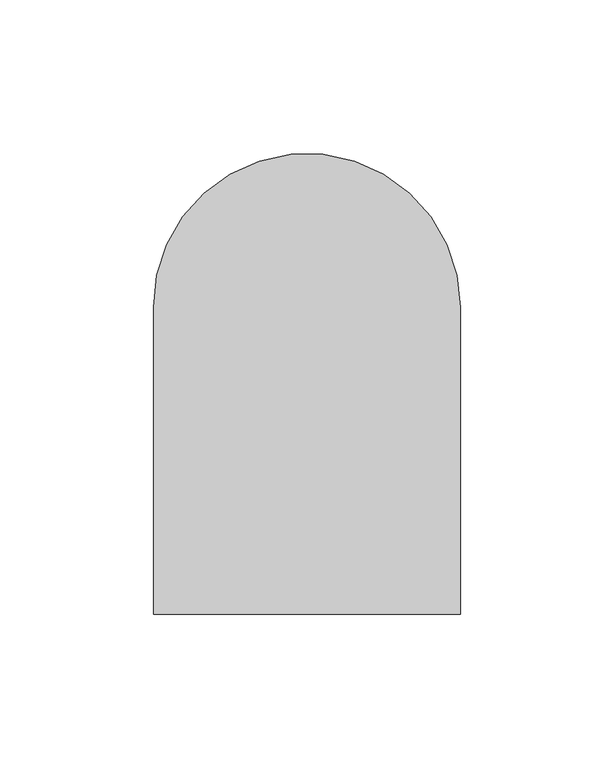
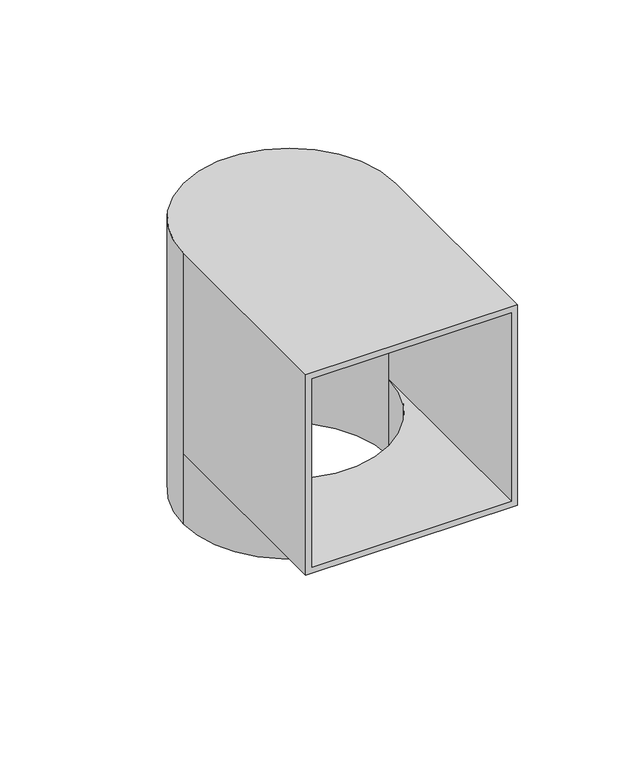
"""IFC4 building model written with IfcOpenShell, lengths in millimetres: proxy geometry, TN_Отвод угловой ТехноНИКОЛЬ : Отвод угловой, с квадратного сечения (100*100мм) в круглое (100мм)."""

import ifcopenshell
import ifcopenshell.guid

model = None  # the IFC model being written
_history = None  # IfcOwnerHistory: only IFC2X3 demands one
_inside = {}  # id of a spatial element -> (the spatial element, [elements in it])
_under = {}  # id of a project, library or spatial element -> (it, [spatial elements below it])
_declared = {}  # id of a project -> (the project, [libraries it declares])
_typed = {}  # id of a type object -> (the type object, [elements of that type])
_made_of = {}  # id of a material, layer set ... -> (it, [elements and type objects made of it])


def new_model(schema):
    """Start an empty IFC model of exactly this schema.

    Asked for "IFC4X3", IfcOpenShell would pick the latest addendum, in which some entities
    have other attributes; the version numbers below select the first issue.
    IFC2X3 requires an IfcOwnerHistory on every rooted entity: one is made here for all.
    """
    global model, _history
    if schema == "IFC4X3":
        model = ifcopenshell.file(schema_version=(4, 3, 0, 0))
    else:
        model = ifcopenshell.file(schema=schema)
    _inside.clear()
    _under.clear()
    _declared.clear()
    _typed.clear()
    _made_of.clear()
    _history = None
    if model.schema == "IFC2X3":
        org = make("IfcOrganization", Name="unknown")
        user = make(
            "IfcPersonAndOrganization",
            ThePerson=make("IfcPerson", FamilyName="unknown"),
            TheOrganization=org,
        )
        app = make(
            "IfcApplication",
            ApplicationDeveloper=org,
            Version="unknown",
            ApplicationFullName="unknown",
            ApplicationIdentifier="unknown",
        )
        _history = make(
            "IfcOwnerHistory",
            OwningUser=user,
            OwningApplication=app,
            ChangeAction="ADDED",
            CreationDate=0,
        )
    return model


def make(cls, **values):
    """One entity of the class cls with the attributes given. An attribute that is None is left unset."""
    return model.create_entity(
        cls, **{name: value for name, value in values.items() if value is not None}
    )


def rooted(cls, **values):
    """An entity with a GlobalId (a new one), such as an element, a storey or a relation."""
    return make(cls, GlobalId=ifcopenshell.guid.new(), OwnerHistory=_history, **values)


def si_unit(unit_type, name, prefix=None):
    """IfcSIUnit, for example si_unit("LENGTHUNIT", "METRE", prefix="MILLI")."""
    return make("IfcSIUnit", UnitType=unit_type, Prefix=prefix, Name=name)


def assignment(units):
    """IfcUnitAssignment: the units of a project."""
    return None if units is None else make("IfcUnitAssignment", Units=units)


def point(xyz):
    """IfcCartesianPoint."""
    return None if xyz is None else make("IfcCartesianPoint", Coordinates=xyz)


def direction(xyz):
    """IfcDirection."""
    return None if xyz is None else make("IfcDirection", DirectionRatios=xyz)


def frame(location, z_axis=None, x_axis=None):
    """IfcAxis2Placement3D, a coordinate frame: its origin and axes. An axis left out is left unset."""
    return make(
        "IfcAxis2Placement3D",
        Location=point(location),
        Axis=direction(z_axis),
        RefDirection=direction(x_axis),
    )


def origin():
    """The frame at (0, 0, 0) with its axes left unset."""
    return frame((0.0, 0.0, 0.0))


def origin_with_axes():
    """The frame at (0, 0, 0) with the z axis (0, 0, 1) and the x axis (1, 0, 0) written out."""
    return frame((0.0, 0.0, 0.0), z_axis=(0.0, 0.0, 1.0), x_axis=(1.0, 0.0, 0.0))


def place(relative_to, where):
    """IfcLocalPlacement: puts the frame where relative to a parent placement (None: the world)."""
    return make(
        "IfcLocalPlacement", PlacementRelTo=relative_to, RelativePlacement=where
    )


def context(
    kind, dimensions, precision=None, world=None, true_north=None, identifier=None
):
    """IfcGeometricRepresentationContext, for example the 3D "Model" context."""
    return make(
        "IfcGeometricRepresentationContext",
        ContextIdentifier=identifier,
        ContextType=kind,
        CoordinateSpaceDimension=dimensions,
        Precision=precision,
        WorldCoordinateSystem=world,
        TrueNorth=true_north,
    )


def project(units=None, contexts=None):
    """IfcProject with its units and contexts."""
    return rooted(
        "IfcProject",
        Name="project",
        RepresentationContexts=contexts,
        UnitsInContext=assignment(units),
    )


def spatial(cls, under=None, at=None, **own):
    """A site, building, storey or space (cls), placed at a placement, below another one or the project."""
    s = rooted(cls, ObjectPlacement=at, **own)
    if under is not None:
        _under.setdefault(under.id(), (under, []))[1].append(s)
    return s


def polyline(points):
    """IfcPolyline through the points."""
    return make("IfcPolyline", Points=[point(p) for p in points])


def circle_curve(where, radius):
    """IfcCircle in the frame where."""
    return make("IfcCircle", Position=where, Radius=radius)


def shape(context_of_items, identifier, shape_type, items):
    """IfcShapeRepresentation: the items that make up one representation, for example the "Body"."""
    return make(
        "IfcShapeRepresentation",
        ContextOfItems=context_of_items,
        RepresentationIdentifier=identifier,
        RepresentationType=shape_type,
        Items=items,
    )


def source(mapping_origin, context_of_items, identifier, shape_type, items):
    """IfcRepresentationMap: a shape defined once, which mapped items show again and again."""
    return make(
        "IfcRepresentationMap",
        MappingOrigin=mapping_origin,
        MappedRepresentation=shape(context_of_items, identifier, shape_type, items),
    )


def transform(
    local_origin,
    x_axis=None,
    y_axis=None,
    z_axis=None,
    scale=None,
    scale2=None,
    scale3=None,
    uniform=True,
):
    """IfcCartesianTransformationOperator3D, or its non-uniform kind. x_axis, y_axis, z_axis: its Axis1, 2, 3."""
    if uniform:
        return make(
            "IfcCartesianTransformationOperator3D",
            Axis1=direction(x_axis),
            Axis2=direction(y_axis),
            LocalOrigin=point(local_origin),
            Scale=scale,
            Axis3=direction(z_axis),
        )
    return make(
        "IfcCartesianTransformationOperator3DnonUniform",
        Axis1=direction(x_axis),
        Axis2=direction(y_axis),
        LocalOrigin=point(local_origin),
        Scale=scale,
        Axis3=direction(z_axis),
        Scale2=scale2,
        Scale3=scale3,
    )


def mapped(mapping_source, mapping_target):
    """IfcMappedItem: shows the shape of a source again, moved by a transform."""
    return make(
        "IfcMappedItem", MappingSource=mapping_source, MappingTarget=mapping_target
    )


def made_of(thing, what):
    """Note that an element or type object is made of a material, layer set ...; save() writes the relation."""
    if what is not None:
        _made_of.setdefault(what.id(), (what, []))[1].append(thing)
    return thing


def element(
    cls,
    number,
    at=None,
    inside=None,
    cuts=None,
    type_object=None,
    material=None,
    context=None,
    identifier="Body",
    shape_type=None,
    held_by="IfcProductDefinitionShape",
    body=None,
    shapes=None,
    **own,
):
    """One element of the class cls, such as IfcWall. Its Tag is "e" and its number.

    at: its placement. inside: the storey or other place that contains it. cuts: it is an
    opening in that element (IfcRelVoidsElement). A single representation is given by context,
    identifier, shape_type and body (its items); several are given by shapes. held_by: the class
    of the entity that holds the representations. save() writes the other relations.
    """
    e = rooted(cls, Tag="e%d" % number, ObjectPlacement=at, **own)
    if body is not None:
        shapes = [shape(context, identifier, shape_type, body)]
    if shapes is not None:
        e.Representation = make(held_by, Representations=shapes)
    if inside is not None:
        _inside.setdefault(inside.id(), (inside, []))[1].append(e)
    if cuts is not None:
        rooted(
            "IfcRelVoidsElement", RelatingBuildingElement=cuts, RelatedOpeningElement=e
        )
    if type_object is not None:
        _typed.setdefault(type_object.id(), (type_object, []))[1].append(e)
    return made_of(e, material)


def aggregate(whole, parts):
    """IfcRelAggregates: a whole, such as a stair, and the parts it consists of."""
    return rooted("IfcRelAggregates", RelatingObject=whole, RelatedObjects=parts)


def save(model, path):
    """Write the relations noted so far, then the file.

    IfcRelAggregates (storeys below a building ...), IfcRelContainedInSpatialStructure (elements
    in a storey), IfcRelDefinesByType, IfcRelAssociatesMaterial and IfcRelDeclares: one each for
    every whole, place, type object, material and project.
    """
    for whole, parts in _under.values():
        aggregate(whole, parts)
    for where, things in _inside.values():
        rooted(
            "IfcRelContainedInSpatialStructure",
            RelatedElements=things,
            RelatingStructure=where,
        )
    for kind, things in _typed.values():
        rooted("IfcRelDefinesByType", RelatedObjects=things, RelatingType=kind)
    for what, things in _made_of.values():
        rooted("IfcRelAssociatesMaterial", RelatedObjects=things, RelatingMaterial=what)
    for by, libraries in _declared.values():
        rooted("IfcRelDeclares", RelatingContext=by, RelatedDefinitions=libraries)
    model.write(path)


def plane_surface(at):
    """IfcPlane: the flat surface through the origin of the frame at, square to its z axis."""
    return make("IfcPlane", Position=at)


def cylinder_surface(at, radius):
    """IfcCylindricalSurface: all points at the distance radius from the z axis of the frame at."""
    return make("IfcCylindricalSurface", Position=at, Radius=radius)


def revolved_surface(curve, axis_point, axis_direction):
    """IfcSurfaceOfRevolution: the curve turned about the line through axis_point along axis_direction."""
    return make(
        "IfcSurfaceOfRevolution",
        SweptCurve=make("IfcArbitraryOpenProfileDef", ProfileType="CURVE", Curve=curve),
        AxisPosition=make("IfcAxis1Placement", Location=point(axis_point), Axis=direction(axis_direction)),
    )


def advanced_brep(points, edges, surfaces, faces):
    """IfcAdvancedBrep: a solid bounded by faces that lie on surfaces and meet in shared edges.

    An edge is (start, end): straight between two places in points (the first is 0);
    or (start, end, curve); or (start, end, curve, False) where it runs against its curve.
    A face is (place in surfaces, loops), or (place, loops, False) where it looks against
    its surface's normal. A loop lists edges by number (the first is 1), with a minus sign
    where the edge is run from its end to its start. The first loop is the outer one.
    """
    corners = [point(p) for p in points]
    vertices = [make("IfcVertexPoint", VertexGeometry=c) for c in corners]
    made = []
    for start, end, *more in edges:
        made.append(
            make(
                "IfcEdgeCurve",
                EdgeStart=vertices[start],
                EdgeEnd=vertices[end],
                EdgeGeometry=more[0] if more else make("IfcPolyline", Points=[corners[start], corners[end]]),
                SameSense=more[1] if len(more) > 1 else True,
            )
        )
    hull = []
    for where, loops, *sense in faces:
        bounds = []
        for j, loop in enumerate(loops):
            ring = [make("IfcOrientedEdge", EdgeElement=made[abs(k) - 1], Orientation=k > 0) for k in loop]
            bounds.append(
                make(
                    "IfcFaceOuterBound" if j == 0 else "IfcFaceBound",
                    Bound=make("IfcEdgeLoop", EdgeList=ring),
                    Orientation=True,
                )
            )
        hull.append(make("IfcAdvancedFace", Bounds=bounds, FaceSurface=surfaces[where], SameSense=sense[0] if sense else True))
    return make("IfcAdvancedBrep", Outer=make("IfcClosedShell", CfsFaces=hull))


def specialty_equipment_3146d892(model_context):
    return source(origin(), model_context, "Body", "AdvancedBrep", [
        advanced_brep(
        [(50.0, -100.0, 0.0), (50.0, -100.0, 100.0), (-50.0, -100.0, 100.0), (-50.0, -100.0, 0.0), (47.0, -100.0, 3.0), (-47.0, -100.0, 3.0), (-47.0, -100.0, 97.0), (47.0, -100.0, 97.0), (50.0, 0.0, 0.0), (50.0, 0.0, 100.0), (-50.0, 0.0, 100.0), (-50.0, 0.0, 0.0), (47.0, 0.0, 3.0), (-47.0, 0.0, 3.0), (-47.0, 0.0, 97.0), (47.0, 0.0, 97.0), (-50.0, 0.0, -35.0), (50.0, 0.0, -35.0), (-47.0, 0.0, -35.0), (47.0, 0.0, -35.0)],
        [
            (0, 1),
            (1, 2),
            (2, 3),
            (3, 0),
            (4, 5),
            (5, 6),
            (6, 7),
            (7, 4),
            (0, 8),
            (8, 9),
            (9, 1),
            (9, 10, circle_curve(frame((0.0, 0.0, 100.0), z_axis=(0.0, 0.0, 1.0), x_axis=(1.0, 0.0, 0.0)), 50.0)),
            (10, 2),
            (10, 11),
            (11, 3),
            (11, 8, circle_curve(origin_with_axes(), 50.0)),
            (4, 12),
            (12, 13, circle_curve(frame((0.0, 0.0, 3.0), z_axis=(0.0, 0.0, -1.0), x_axis=(1.0, 0.0, 0.0)), 47.0)),
            (13, 5),
            (13, 14),
            (14, 6),
            (14, 15, circle_curve(frame((0.0, 0.0, 97.0), z_axis=(0.0, 0.0, -1.0), x_axis=(1.0, 0.0, 0.0)), 47.0)),
            (15, 7),
            (15, 12),
            (16, 17, circle_curve(frame((0.0, 0.0, -35.0), z_axis=(0.0, 0.0, -1.0), x_axis=(1.0, 0.0, 0.0)), 50.0)),
            (17, 16, circle_curve(frame((0.0, 0.0, -35.0), z_axis=(0.0, 0.0, -1.0), x_axis=(1.0, 0.0, 0.0)), 50.0)),
            (18, 19, circle_curve(frame((0.0, 0.0, -35.0), z_axis=(0.0, 0.0, 1.0), x_axis=(1.0, 0.0, 0.0)), 47.0)),
            (19, 18, circle_curve(frame((0.0, 0.0, -35.0), z_axis=(0.0, 0.0, 1.0), x_axis=(1.0, 0.0, 0.0)), 47.0)),
            (17, 8),
            (11, 16),
            (18, 13),
            (12, 19),
        ],
        [
            plane_surface(frame((-50.0, -100.0, 0.0), z_axis=(0.0, -1.0, 0.0), x_axis=(1.0, 0.0, 0.0))),
            plane_surface(frame((50.0, 0.0, 100.0), z_axis=(1.0, 0.0, 0.0), x_axis=(0.0, -1.0, 0.0))),
            plane_surface(frame((-50.0, 0.0, 100.0), z_axis=(0.0, 0.0, 1.0), x_axis=(0.0, -1.0, 0.0))),
            plane_surface(frame((-50.0, 0.0, 0.0), z_axis=(-1.0, 0.0, 0.0), x_axis=(0.0, -1.0, 0.0))),
            plane_surface(frame((50.0, 0.0, 0.0), z_axis=(0.0, 0.0, -1.0), x_axis=(0.0, -1.0, 0.0))),
            plane_surface(frame((-47.0, 0.0, 3.0), z_axis=(0.0, 0.0, 1.0), x_axis=(0.0, -1.0, 0.0))),
            plane_surface(frame((-47.0, 0.0, 97.0), z_axis=(1.0, 0.0, 0.0), x_axis=(0.0, -1.0, 0.0))),
            plane_surface(frame((47.0, 0.0, 97.0), z_axis=(0.0, 0.0, -1.0), x_axis=(0.0, -1.0, 0.0))),
            plane_surface(frame((47.0, 0.0, 3.0), z_axis=(-1.0, 0.0, 0.0), x_axis=(0.0, -1.0, 0.0))),
            plane_surface(frame((50.0, 0.0, -35.0), z_axis=(0.0, 0.0, -1.0), x_axis=(0.0, -1.0, 0.0))),
            cylinder_surface(frame((0.0, 0.0, -35.0), z_axis=(0.0, 0.0, 1.0), x_axis=(1.0, 0.0, 0.0)), 50.0),
            revolved_surface(polyline([(47.0, 0.0, 3.0), (47.0, 0.0, -35.0)]), (0.0, 0.0, -35.0), (0.0, 0.0, 1.0)),
            revolved_surface(polyline([(47.0, 0.0, 97.0), (47.0, 0.0, -35.0)]), (0.0, 0.0, -35.0), (0.0, 0.0, 1.0)),
        ],
        [
            (0, [[1, 2, 3, 4], [5, 6, 7, 8]]),
            (1, [[-1, 9, 10, 11]]),
            (2, [[-2, -11, 12, 13]]),
            (3, [[-3, -13, 14, 15]]),
            (4, [[-4, -15, 16, -9]]),
            (5, [[-5, 17, 18, 19]]),
            (6, [[-6, -19, 20, 21]]),
            (7, [[-7, -21, 22, 23]]),
            (8, [[-17, -8, -23, 24]]),
            (9, [[25, 26], [27, 28]]),
            (10, [[-26, 29, -16, 30]]),
            (10, [[-12, -10, -29, -25, -30, -14]]),
            (11, [[-27, 31, -18, 32]]),
            (12, [[-22, -20, -31, -28, -32, -24]]),
        ],
    ),
    ])


if __name__ == "__main__":
    model = new_model("IFC4")
    model_context = context("Model", 3, world=origin())
    ifc_project = project(units=[si_unit("LENGTHUNIT", "METRE", prefix="MILLI")], contexts=[model_context])
    site = spatial("IfcSite", under=ifc_project)
    building = spatial("IfcBuilding", under=site)
    placement = place(None, origin())
    specialty_equipment_shape = specialty_equipment_3146d892(model_context)
    element("IfcBuildingElementProxy", 1, Name="TN_Отвод угловой ТехноНИКОЛЬ : Отвод угловой, с квадратного сечения (100*100мм) в круглое (100мм)", ObjectType="TN_Отвод угловой ТехноНИКОЛЬ : Отвод угловой, с квадратного сечения (100*100мм) в круглое (100мм)", at=placement, inside=building, context=model_context, shape_type="MappedRepresentation", body=[
        mapped(specialty_equipment_shape, transform((0.0, 0.0, 0.0), x_axis=(1.0, 0.0, 0.0), y_axis=(0.0, 1.0, 0.0), z_axis=(0.0, 0.0, 1.0))),
    ])
    save(model, "model.ifc")

# Revit data of these elements
# Type "TN_Отвод угловой ТехноНИКОЛЬ : Отвод угловой, с квадратного сечения (100*100мм) в круглое (100мм)"
#   ADSK_Группирование = "Комплектующие и воронки"
#   Description = "Угловой соединительный элемент служит для отвода дождевой воды из парапетных воронок, расположенных горизонтально, в вертикальные водостоки. Внутренние рёбра позволяют отличное закрепление патрубков, предотвращая любые деформации со временем. Угловой соединительный элемент изготавливается из полипропилена (черный), устойчивого к воздействию низких температур."
#   Manufacturer = "ТехноНИКОЛЬ"
#   URL = "https://www.tstn.ru/product/otvod-uglovoy-plastikovyy-diametr-100mm-100-100mm/"
#   ADSK_Примечание [instance default] = ""
#   ADSK_Обозначение = "ТехноНИКОЛЬ"
#   ADSK_Наименование = "Отвод угловой, с квадратного сечения (100*100мм) в круглое (100мм)"
#   ADSK_Марка = ""
#   ADSK_Код изделия = "660284"
#   ADSK_Завод-изготовитель = "ТехноНИКОЛЬ"
#   ADSK_Единица измерения = "шт."
#   ADSK_Группирование = "Комплектующие и воронки"
#   ADSK_URL страницы изделия = "https://www.tstn.ru/product/otvod-uglovoy-plastikovyy-diametr-100mm-100-100mm/"
#   ADSK_URL документации изделия = ""
#   ADSK_Размер_Ширина = 100 mm
#   ADSK_Размер_Высота = 100 mm
#   ADSK_Количество = 1
#   Видимость_Переход [instance default] = yes
#   ADSK_Материал [instance default] = TN_ПВХ_Черный
#   Default Elevation = 0
# Element 1 (IfcBuildingElementProxy, "TN_Отвод угловой ТехноНИКОЛЬ : Отвод угловой, с квадратного сечения (100*100мм) в круглое (100мм)")
#   Materials on its faces: "TN_ПВХ_Черный"
# Materials
#   "TN_ПВХ_Черный": class "Типовые", colour RGB 48 48 48, transparency 0, Cost = 0
